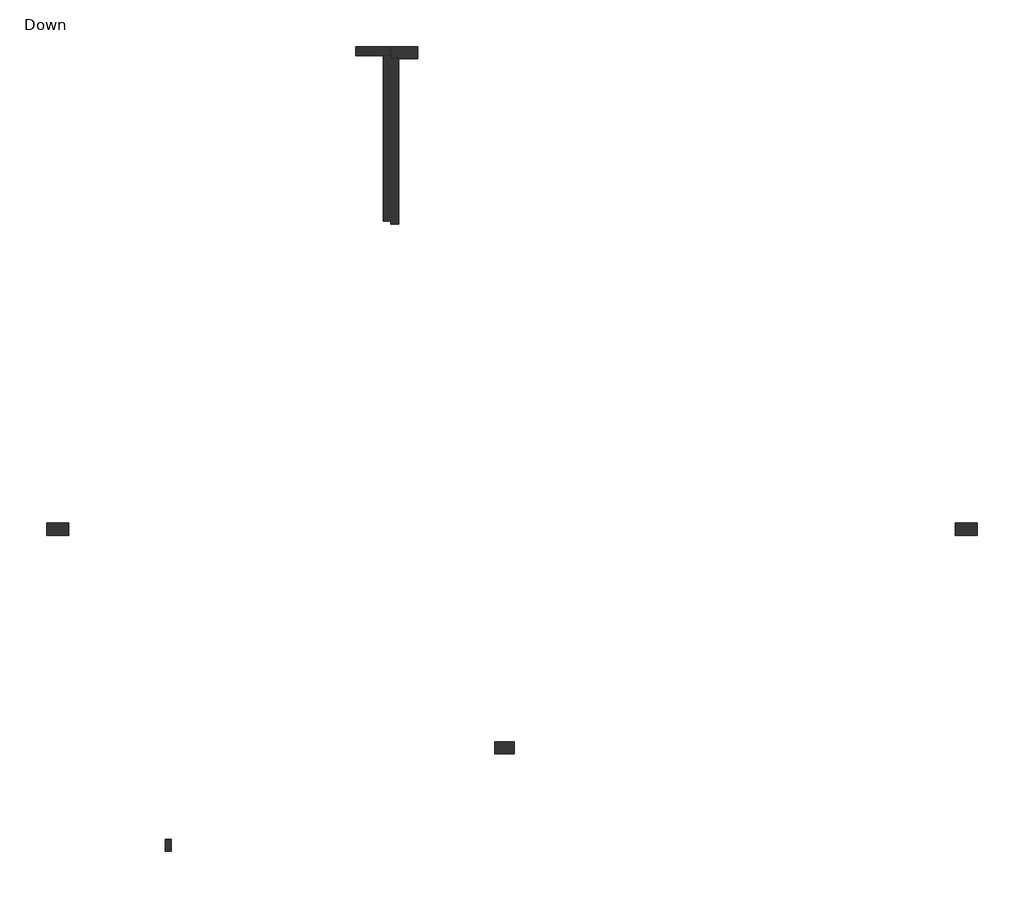
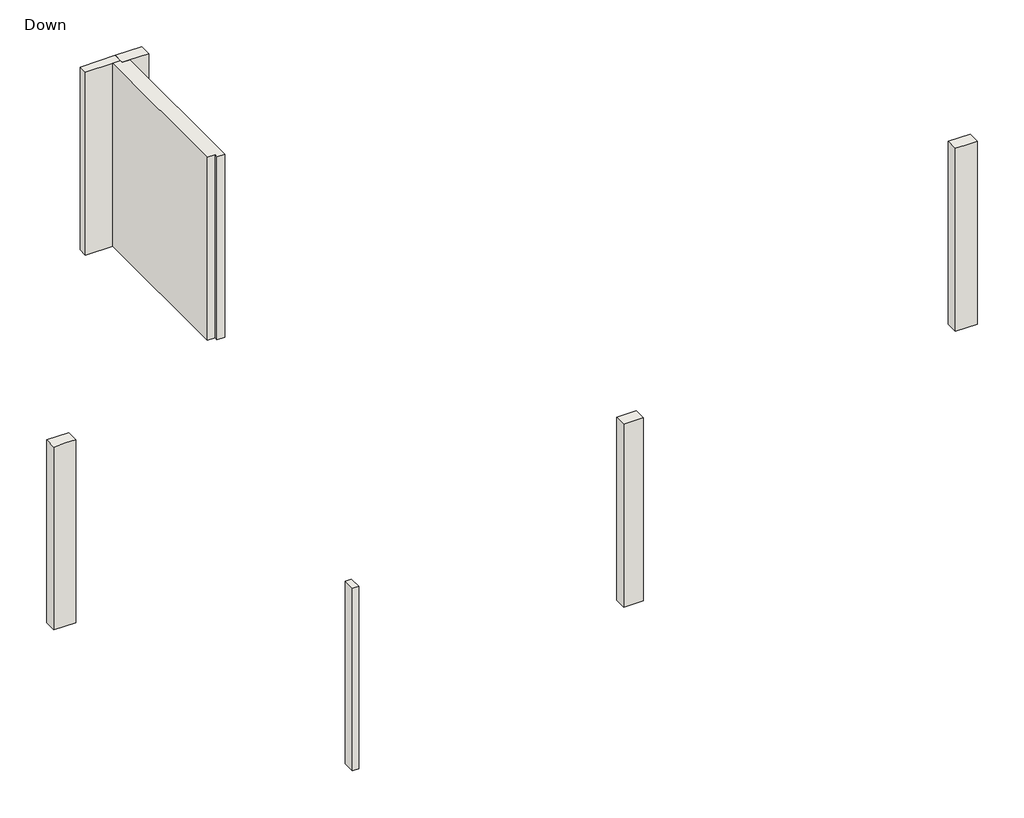
# One storey: 7 walls.
"""IFC4 building model written with IfcOpenShell, lengths in millimetres."""

from ifc_helpers import new_model, si_unit, origin, place, context, project, spatial, faceted_brep, element, save

model = new_model("IFC4")

# Units and contexts
model_context = context("Model", 3, world=origin())
ifc_project = project(units=[si_unit("LENGTHUNIT", "METRE", prefix="MILLI")], contexts=[model_context])

# Site, building, storey
site = spatial("IfcSite", under=ifc_project)
building = spatial("IfcBuilding", under=site)
storey = spatial("IfcBuildingStorey", under=building, Name="Down", Elevation=0.0)

# Walls
placement = place(None, origin())
element("IfcWall", 1, ObjectType="15", at=placement, inside=storey, context=model_context, shape_type="Brep", body=[
    faceted_brep([(2556.6955539, 306.3601755, 0.0), (1986.6955539, 306.3601755, 0.0), (1986.6955539, 306.3601755, 2810.0), (1986.6955539, 306.3601755, 3010.0), (1986.6955539, 306.3601755, 3160.0), (2556.6955539, 306.3601755, 3160.0), (2556.6955539, 156.3601755, 0.0), (2556.6955539, 156.3601755, 3160.0), (2431.6955539, 156.3601755, 3160.0), (1986.6955539, 156.3601755, 3160.0), (1986.6955539, 156.3601755, 3010.0), (1986.6955539, 156.3601755, 2810.0), (1986.6955539, 156.3601755, 0.0), (2431.6955539, 156.3601755, 0.0)], [[[0, 1, 2, 3, 4, 5]], [[6, 7, 8, 9, 10, 11, 12, 13]], [[1, 0, 6, 13, 12]], [[4, 3, 2, 1, 12, 11, 10, 9]], [[5, 4, 9, 8, 7]], [[0, 5, 7, 6]]]),
])
element("IfcWall", 2, ObjectType="20", at=placement, inside=storey, context=model_context, shape_type="Brep", body=[
    faceted_brep([(2556.6955539, 106.3601755, 0.0), (2681.6955539, 106.3601755, 0.0), (2996.6955539, 106.3601755, 0.0), (2996.6955539, 106.3601755, 2810.0), (2996.6955539, 106.3601755, 3010.0), (2996.6955539, 106.3601755, 3160.0), (2681.6955539, 106.3601755, 3160.0), (2556.6955539, 106.3601755, 3160.0), (2556.6955539, 306.3601755, 0.0), (2556.6955539, 306.3601755, 3160.0), (2996.6955539, 306.3601755, 3160.0), (2996.6955539, 306.3601755, 3010.0), (2996.6955539, 306.3601755, 2810.0), (2996.6955539, 306.3601755, 0.0), (2556.6955539, 156.3601755, 0.0), (2556.6955539, 156.3601755, 3160.0)], [[[0, 1, 2, 3, 4, 5, 6, 7]], [[8, 9, 10, 11, 12, 13]], [[2, 1, 0, 14, 8, 13]], [[5, 4, 3, 2, 13, 12, 11, 10]], [[7, 6, 5, 10, 9, 15]], [[0, 7, 15, 9, 8, 14]]]),
])
element("IfcWall", 3, ObjectType="20", at=placement, inside=storey, context=model_context, shape_type="Brep", body=[
    faceted_brep([(-1004.0660316, -12552.855147, 0.0), (-1104.0660316, -12552.855147, 0.0), (-1104.0660316, -12552.855147, 2810.0), (-1104.0660316, -12552.855147, 3010.0), (-1104.0660316, -12552.855147, 3160.0), (-1004.0660316, -12552.855147, 3160.0), (-1004.0660316, -12552.855147, 3010.0), (-1004.0660316, -12552.855147, 2810.0), (-1004.0660316, -12752.855147, 0.0), (-1004.0660316, -12752.855147, 3160.0), (-1104.0660316, -12752.855147, 3160.0), (-1104.0660316, -12752.855147, 0.0)], [[[0, 1, 2, 3, 4, 5, 6, 7]], [[8, 9, 10, 11]], [[1, 0, 8, 11]], [[5, 4, 10, 9]], [[0, 7, 6, 5, 9, 8]], [[4, 3, 2, 1, 11, 10]]]),
])
element("IfcWall", 4, ObjectType="20", at=placement, inside=storey, context=model_context, shape_type="Brep", body=[
    faceted_brep([(-2665.7294994, -7425.251138, 0.0), (-3025.7294994, -7425.251138, 0.0), (-3025.7294994, -7425.251138, 2810.0), (-3025.7294994, -7425.251138, 3010.0), (-3025.7294994, -7425.251138, 3160.0), (-2665.7294994, -7425.251138, 3160.0), (-2665.7294994, -7425.251138, 3010.0), (-2665.7294994, -7425.251138, 2810.0), (-2665.7294994, -7625.251138, 0.0), (-2665.7294994, -7625.251138, 2810.0), (-2665.7294994, -7625.251138, 3010.0), (-2665.7294994, -7625.251138, 3160.0), (-2825.7294994, -7625.251138, 3160.0), (-3025.7294994, -7625.251138, 3160.0), (-3025.7294994, -7625.251138, 160.0), (-3025.7294994, -7625.251138, 0.0)], [[[0, 1, 2, 3, 4, 5, 6, 7]], [[8, 9, 10, 11, 12, 13, 14, 15]], [[1, 0, 8, 15]], [[5, 4, 13, 12, 11]], [[0, 7, 6, 5, 11, 10, 9, 8]], [[4, 3, 2, 1, 15, 14, 13]]]),
])
element("IfcWall", 5, ObjectType="20", at=placement, inside=storey, context=model_context, shape_type="Brep", body=[
    faceted_brep([(4561.3412033, -10973.6256761, 0.0), (4241.3412033, -10973.6256761, 0.0), (4241.3412033, -10973.6256761, 2810.0), (4241.3412033, -10973.6256761, 3010.0), (4241.3412033, -10973.6256761, 3160.0), (4561.3412033, -10973.6256761, 3160.0), (4561.3412033, -10973.6256761, 3010.0), (4561.3412033, -10973.6256761, 2810.0), (4561.3412033, -11173.6256761, 0.0), (4561.3412033, -11173.6256761, 2810.0), (4561.3412033, -11173.6256761, 3010.0), (4561.3412033, -11173.6256761, 3160.0), (4441.3412033, -11173.6256761, 3160.0), (4241.3412033, -11173.6256761, 3160.0), (4241.3412033, -11173.6256761, 160.0), (4241.3412033, -11173.6256761, 0.0)], [[[0, 1, 2, 3, 4, 5, 6, 7]], [[8, 9, 10, 11, 12, 13, 14, 15]], [[1, 0, 8, 15]], [[5, 4, 13, 12, 11]], [[0, 7, 6, 5, 11, 10, 9, 8]], [[4, 3, 2, 1, 15, 14, 13]]]),
])
element("IfcWall", 6, ObjectType="20", at=placement, inside=storey, context=model_context, shape_type="Brep", body=[
    faceted_brep([(12069.8374389, -7425.251138, 0.0), (11709.8374389, -7425.251138, 0.0), (11709.8374389, -7425.251138, 2810.0), (11709.8374389, -7425.251138, 3010.0), (11709.8374389, -7425.251138, 3160.0), (12069.8374389, -7425.251138, 3160.0), (12069.8374389, -7425.251138, 3010.0), (12069.8374389, -7425.251138, 2810.0), (12069.8374389, -7625.251138, 0.0), (12069.8374389, -7625.251138, 160.0), (12069.8374389, -7625.251138, 3160.0), (11869.8374389, -7625.251138, 3160.0), (11709.8374389, -7625.251138, 3160.0), (11709.8374389, -7625.251138, 3010.0), (11709.8374389, -7625.251138, 2810.0), (11709.8374389, -7625.251138, 0.0)], [[[0, 1, 2, 3, 4, 5, 6, 7]], [[8, 9, 10, 11, 12, 13, 14, 15]], [[1, 0, 8, 15]], [[4, 3, 2, 1, 15, 14, 13, 12]], [[5, 4, 12, 11, 10]], [[0, 7, 6, 5, 10, 9, 8]]]),
])
element("IfcWall", 7, ObjectType="25", at=placement, inside=storey, context=model_context, shape_type="Brep", body=[
    faceted_brep([(2431.6955539, 156.3601755, 0.0), (2431.6955539, -2526.1363023, 0.0), (2431.6955539, -2526.1363023, 2810.0), (2431.6955539, -2526.1363023, 3010.0), (2431.6955539, -2526.1363023, 3160.0), (2431.6955539, 156.3601755, 3160.0), (2431.6955539, 156.3601755, 3010.0), (2431.6955539, 156.3601755, 2810.0), (2681.6955539, 106.3601755, 0.0), (2681.6955539, 106.3601755, 3160.0), (2681.6955539, -2576.1363023, 3160.0), (2681.6955539, -2576.1363023, 0.0), (2556.6955539, 156.3601755, 0.0), (2556.6955539, 106.3601755, 0.0), (2556.6955539, -2576.1363023, 0.0), (2556.6955539, -2526.1363023, 0.0), (2556.6955539, -2526.1363023, 3160.0), (2556.6955539, -2576.1363023, 3160.0), (2556.6955539, 106.3601755, 3160.0), (2556.6955539, 156.3601755, 3160.0), (2556.6955539, -2526.1363023, 160.0), (2556.6955539, -2576.1363023, 160.0)], [[[0, 1, 2, 3, 4, 5, 6, 7]], [[8, 9, 10, 11]], [[1, 0, 12, 13, 8, 11, 14, 15]], [[5, 4, 16, 17, 10, 9, 18, 19]], [[4, 3, 2, 1, 15, 20, 16]], [[15, 14, 21, 17, 16, 20]], [[14, 11, 10, 17, 21]], [[0, 7, 6, 5, 19, 12]], [[19, 18, 13, 12]], [[18, 9, 8, 13]]]),
])

save(model, "model.ifc")

# Revit data of these elements
# Project information
#   Project Issue Date = "Issue Date"
#   Project Status = "Project Status"
#   Client Name = "לקוח"
#   Project Address = "Enter address here"
#   Project Name = "Project 002"
#   Project Number = "מספר פרויקט"
# Type "15"
#   Layers, outside or top first: 15 cm "Concrete, Cast-in-Place - B30" (function 1)
# Type "20"
#   Layers, outside or top first: 20 cm "Concrete, Cast-in-Place - B30" (function 1)
# Type "25"
#   Layers, outside or top first: 25 cm "Concrete, Cast-in-Place - B30" (function 1)
# Element 1 (IfcWall, "15")
#   Comments = ""
#   Mark = "W104"
#   SOFiSTiK_AMG_Comments = ""
#   Top Offset = 0 cm
#   Base Offset = 0 cm
#   wall height = 316 cm
#   SOFiSTiK_AMG_Scheduled = yes
#   SOFiSTiK_AMG_Adjusted = yes
#   Phase Created = New Construction
#   Base Constraint = Down
#   Top Constraint = Typical Floor
#   Materials on its faces: "Concrete, Cast-in-Place - B30"
# Element 2 (IfcWall, "20")
#   Comments = ""
#   Mark = "W57"
#   SOFiSTiK_AMG_Comments = ""
#   Top Offset = 0 cm
#   Base Offset = 0 cm
#   wall height = 316 cm
#   SOFiSTiK_AMG_Scheduled = yes
#   SOFiSTiK_AMG_Adjusted = yes
#   Phase Created = New Construction
#   Base Constraint = Down
#   Top Constraint = Typical Floor
#   Materials on its faces: "Concrete, Cast-in-Place - B30"
# Element 3 (IfcWall, "20")
#   Comments = ""
#   Mark = "W58"
#   SOFiSTiK_AMG_Comments = "Too Short /"
#   Top Offset = 0 cm
#   Base Offset = 0 cm
#   wall height = 316 cm
#   SOFiSTiK_AMG_Scheduled = yes
#   SOFiSTiK_AMG_Adjusted = yes
#   Phase Created = New Construction
#   Base Constraint = Down
#   Top Constraint = Typical Floor
#   Materials on its faces: "Concrete, Cast-in-Place - B30"
# Element 4 (IfcWall, "20")
#   Comments = ""
#   Mark = "W59"
#   SOFiSTiK_AMG_Comments = ""
#   Top Offset = 0 cm
#   Base Offset = 0 cm
#   wall height = 316 cm
#   SOFiSTiK_AMG_Scheduled = yes
#   SOFiSTiK_AMG_Adjusted = yes
#   Phase Created = New Construction
#   Base Constraint = Down
#   Top Constraint = Typical Floor
#   Materials on its faces: "Concrete, Cast-in-Place - B30"
# Element 5 (IfcWall, "20")
#   Comments = ""
#   Mark = "W60"
#   SOFiSTiK_AMG_Comments = ""
#   Top Offset = 0 cm
#   Base Offset = 0 cm
#   wall height = 316 cm
#   SOFiSTiK_AMG_Scheduled = yes
#   SOFiSTiK_AMG_Adjusted = yes
#   Phase Created = New Construction
#   Base Constraint = Down
#   Top Constraint = Typical Floor
#   Materials on its faces: "Concrete, Cast-in-Place - B30"
# Element 6 (IfcWall, "20")
#   Comments = ""
#   Mark = "W61"
#   SOFiSTiK_AMG_Comments = ""
#   Top Offset = 0 cm
#   Base Offset = 0 cm
#   wall height = 316 cm
#   SOFiSTiK_AMG_Scheduled = yes
#   SOFiSTiK_AMG_Adjusted = yes
#   Phase Created = New Construction
#   Base Constraint = Down
#   Top Constraint = Typical Floor
#   Materials on its faces: "Concrete, Cast-in-Place - B30"
# Element 7 (IfcWall, "25")
#   Comments = ""
#   Mark = "W90"
#   SOFiSTiK_AMG_Comments = ""
#   Top Offset = 0 cm
#   Base Offset = 0 cm
#   wall height = 316 cm
#   SOFiSTiK_AMG_Scheduled = yes
#   SOFiSTiK_AMG_Adjusted = yes
#   Phase Created = New Construction
#   Base Constraint = Down
#   Top Constraint = Typical Floor
#   Materials on its faces: "Concrete, Cast-in-Place - B30"
# Materials
#   "Concrete, Cast-in-Place - B30": class "Concrete", colour RGB 192 192 192, transparency 0, Keynote = "01000", Description = "Cast-in-place concrete", Cost = 0
